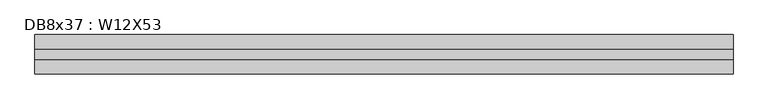
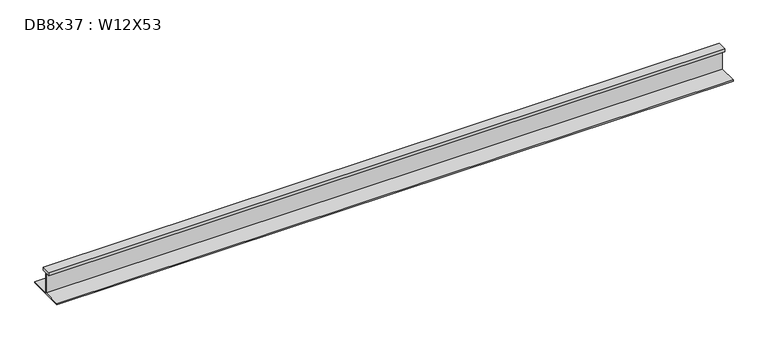
"""IFC4 building model written with IfcOpenShell, lengths in millimetres: beam geometry, DB8x37 : W12X53."""

from ifc_helpers import new_model, si_unit, frame, origin, place, context, project, spatial, polyline, outline, extrude, source, transform, mapped, element, save


def db8x37_w12x53_2f7a65f9(model_context):
    return source(origin(), model_context, "Body", "SweptSolid", [
        extrude(outline(polyline([(38.1, 145.415), (38.1, 120.015), (2.921, 120.015), (2.921, -48.4505), (152.4, -48.4505), (152.4, -58.1025), (-152.4, -58.1025), (-152.4, -48.4505), (-2.921, -48.4505), (-2.921, 120.015), (-38.1, 120.015), (-38.1, 145.415), (38.1, 145.415)])), frame((-2743.2, 0.0, 0.0), z_axis=(1.0, 0.0, 0.0), x_axis=(0.0, 1.0, 0.0)), (0.0, 0.0, 1.0), 5388.229),
    ])


if __name__ == "__main__":
    model = new_model("IFC4")
    model_context = context("Model", 3, world=origin())
    ifc_project = project(units=[si_unit("LENGTHUNIT", "METRE", prefix="MILLI")], contexts=[model_context])
    site = spatial("IfcSite", under=ifc_project)
    building = spatial("IfcBuilding", under=site)
    placement = place(None, origin())
    db8x37_w12x53_shape = db8x37_w12x53_2f7a65f9(model_context)
    element("IfcBeam", 1, ObjectType="DB8x37 : W12X53", at=placement, inside=building, context=model_context, shape_type="MappedRepresentation", body=[
        mapped(db8x37_w12x53_shape, transform((0.0, 0.0, 0.0), x_axis=(1.0, 0.0, 0.0), y_axis=(0.0, 1.0, 0.0), z_axis=(0.0, 0.0, 1.0))),
    ])
    save(model, "model.ifc")

# Revit data of these elements
# Type "DB8x37 : W12X53"
#   Assembly Code = "B10"
#   W = 53
#   Length [instance default] = 5' - 0"
#   bf = 0' - 10"
#   d = 1' - 0.1"
#   k = 0' - 1 3/8"
#   k2 = 0' - 0.8"
#   tf = 0' - 0.575"
#   tw = 0' - 0.345"
#   A = 0.108333 SF
#   Structural Material [instance default] = Steel ASTM A992
# Element 1 (IfcBeam, "DB8x37 : W12X53")
#   Materials on its faces: "Steel ASTM A992"
# Materials
#   "Steel ASTM A992": class "Metal", colour RGB 199 199 199, transparency 0, Description = "Structural steel 50ksi", Cost = 0
